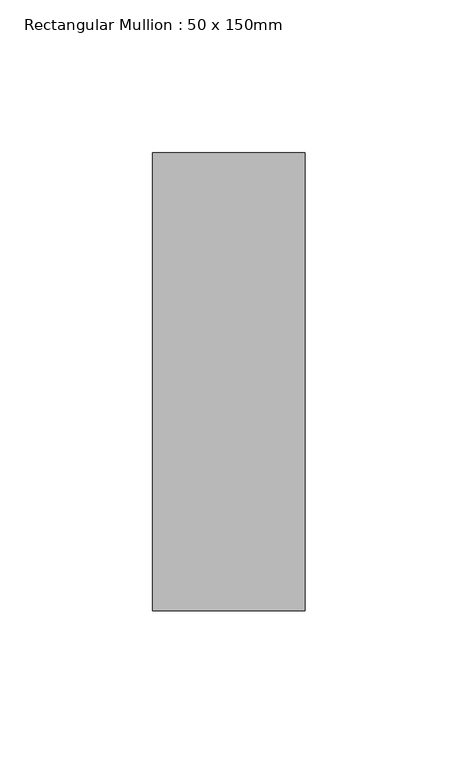
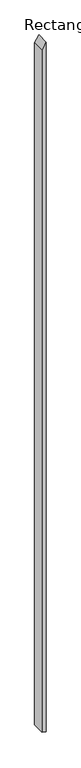
"""IFC4 building model written with IfcOpenShell, lengths in millimetres: member geometry, Rectangular Mullion : 50 x 150mm."""

from ifc_helpers import new_model, si_unit, frame, origin, place, context, project, spatial, polyline, outline, extrude, source, transform, mapped, element, save


def rectangular_mullion_50_x_150mm_d07257d7(model_context):
    return source(origin(), model_context, "Body", "SweptSolid", [
        extrude(outline(polyline([(0.0, 0.0), (-83.6497392, -50.0), (-8698.3621073, -50.0), (-8710.0715519, 0.0), (0.0, 0.0)])), frame((0.0, -75.0, 0.0), z_axis=(0.0, 1.0, 0.0), x_axis=(0.0, 0.0, 1.0)), (0.0, 0.0, 1.0), 150.0),
    ])


if __name__ == "__main__":
    model = new_model("IFC4")
    model_context = context("Model", 3, world=origin())
    ifc_project = project(units=[si_unit("LENGTHUNIT", "METRE", prefix="MILLI")], contexts=[model_context])
    site = spatial("IfcSite", under=ifc_project)
    building = spatial("IfcBuilding", under=site)
    placement = place(None, origin())
    rectangular_mullion_50_x_150mm_shape = rectangular_mullion_50_x_150mm_d07257d7(model_context)
    element("IfcMember", 1, ObjectType="Rectangular Mullion : 50 x 150mm", at=placement, inside=building, context=model_context, shape_type="MappedRepresentation", body=[
        mapped(rectangular_mullion_50_x_150mm_shape, transform((0.0, 0.0, 0.0), x_axis=(1.0, 0.0, 0.0), y_axis=(0.0, 1.0, 0.0), z_axis=(0.0, 0.0, 1.0))),
    ])
    save(model, "model.ifc")

# Revit data of these elements
# Type "Rectangular Mullion : 50 x 150mm"
#   built-in parameter 1007304 = 0.492126 (stored number, unit not read)
#   built-in parameter 1007301 = 0.082021 (stored number, unit not read)
#   built-in parameter 1007300 = 0.082021 (stored number, unit not read)
# Element 1 (IfcMember, "Rectangular Mullion : 50 x 150mm")
#   Materials on its faces: "Metal - Aluminium"
# Materials
#   "Metal - Aluminium": class "Metal", colour RGB 247 247 247, transparency 0
